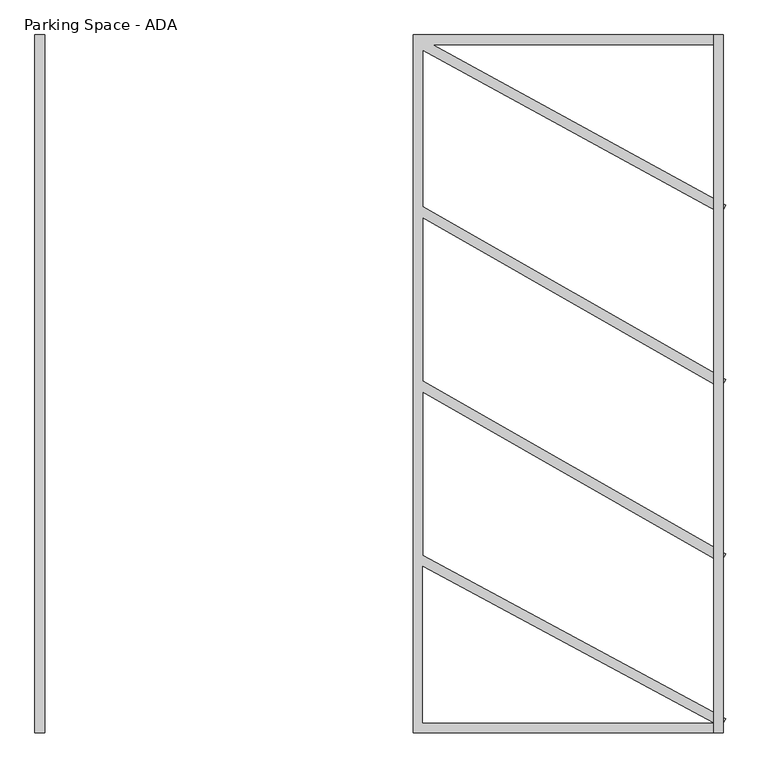
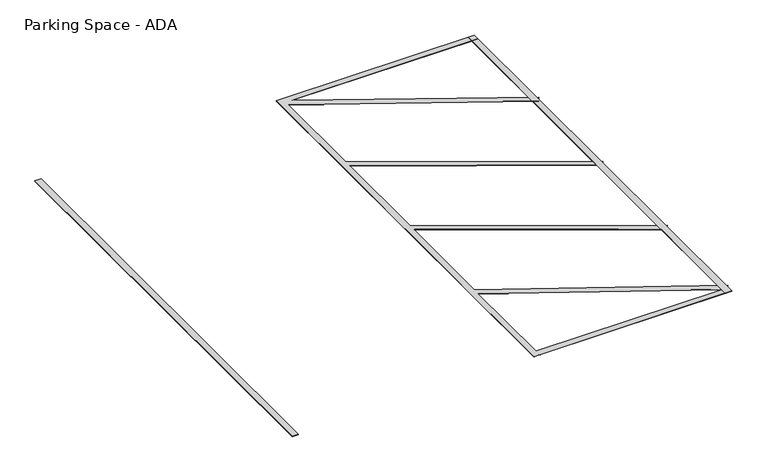
"""IFC4 building model written with IfcOpenShell, lengths in millimetres: proxy geometry, Parking Space - ADA : 9' x 18' (8' Aisle)."""

from ifc_helpers import new_model, si_unit, origin, origin_with_axes, place, context, project, spatial, polyline, outline, extrude, source, transform, mapped, element, save


def parking_space_ada_9beafb2e(model_context):
    return source(origin(), model_context, "Body", "SweptSolid", [
        extrude(outline(polyline([(6637.0620479, -859.2253385), (6560.8620479, -859.2253385), (6560.8620479, 4627.1746615), (6637.0620479, 4627.1746615), (6637.0620479, -859.2253385)])), origin_with_axes(), (0.0, 0.0, 1.0), 1.5875),
        extrude(outline(polyline([(4274.8620479, -859.2253385), (4198.6620479, -859.2253385), (4198.6620479, 4627.1746615), (4274.8620479, 4627.1746615), (6637.0620479, 4627.1746615), (6637.0620479, 4550.9746615), (4354.0996019, 4550.9746615), (6655.3817704, 3288.9812143), (6618.7423254, 3222.1681088), (4274.8620479, 4507.5218093), (4274.8620479, 3277.6849501), (6655.9649414, 1917.0547253), (6618.1591543, 1850.8945978), (4274.8620479, 3189.9215158), (4274.8620479, 1906.0849501), (6655.9649414, 545.4547253), (6618.1591543, 479.2945978), (4274.8620479, 1818.3215158), (4274.8620479, 535.1071205), (6655.15698, -749.4964937), (6637.0620479, -783.0253385), (6637.0620479, -859.2253385), (4274.8620479, -859.2253385)]), holes=[polyline([(6556.8401387, -783.0253385), (4274.8620479, 448.5183931), (4274.8620479, -783.0253385), (6556.8401387, -783.0253385)])]), origin_with_axes(), (0.0, 0.0, 1.0), 1.5875),
        extrude(outline(polyline([(1303.0620479, -859.2253385), (1226.8620479, -859.2253385), (1226.8620479, 4627.1746615), (1303.0620479, 4627.1746615), (1303.0620479, -859.2253385)])), origin_with_axes(), (0.0, 0.0, 1.0), 1.5875),
    ])


if __name__ == "__main__":
    model = new_model("IFC4")
    model_context = context("Model", 3, world=origin())
    ifc_project = project(units=[si_unit("LENGTHUNIT", "METRE", prefix="MILLI")], contexts=[model_context])
    site = spatial("IfcSite", under=ifc_project)
    building = spatial("IfcBuilding", under=site)
    placement = place(None, origin())
    parking_space_ada_shape = parking_space_ada_9beafb2e(model_context)
    element("IfcBuildingElementProxy", 1, Name="Parking Space - ADA : 9' x 18' (8' Aisle)", ObjectType="Parking Space - ADA : 9' x 18' (8' Aisle)", at=placement, inside=building, context=model_context, shape_type="MappedRepresentation", body=[
        mapped(parking_space_ada_shape, transform((0.0, 0.0, 0.0), x_axis=(1.0, 0.0, 0.0), y_axis=(0.0, 1.0, 0.0), z_axis=(0.0, 0.0, 1.0))),
    ])
    save(model, "model.ifc")

# Revit data of these elements
# Type "Parking Space - ADA : 9' x 18' (8' Aisle)"
#   Accesible Aisle = 8' - 0"
#   Length = 18' - 0"
#   Width = 9' - 9"
# Element 1 (IfcBuildingElementProxy, "Parking Space - ADA : 9' x 18' (8' Aisle)")
#   Materials on its faces: "ADA VAN ACCESSIBLE STALL"
# Materials
#   "ADA VAN ACCESSIBLE STALL": class "Paint", colour RGB 255 255 255, transparency 0, Cost = 0
